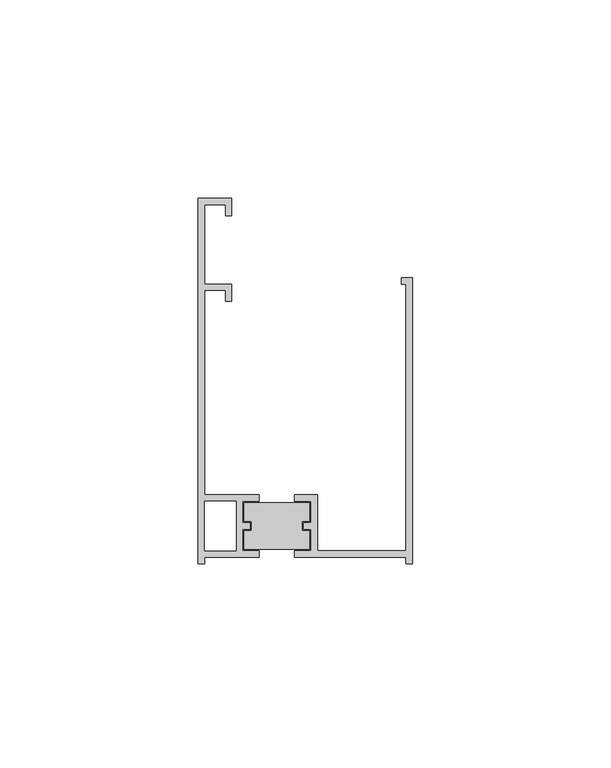
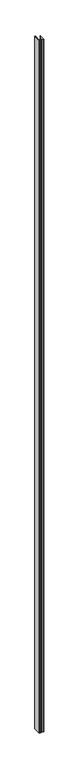
"""IFC4 building model written with IfcOpenShell, lengths in millimetres: proxy geometry, Generic Models 2:Generic Models 2:310765:Generic Models 2:310765 : Generic Models 2:Generic Models 2:310765:60 : Generic Models 2:Generic Models 2:310765:Generic Models 2:310765 : Generic Models 2:Generic Models 2:310765:300385."""

from ifc_helpers import new_model, si_unit, origin, origin_with_axes, place, context, project, spatial, polyline, outline, extrude, source, transform, mapped, element, save


def generic_models_ff3dd308(model_context):
    return source(origin(), model_context, "Body", "SweptSolid", [
        extrude(outline(polyline([(667633.5969099, -465596.2158643), (667633.5969099, -465600.9133629), (667631.6714944, -465600.9133629), (667631.6714944, -465603.2946129), (667633.5969099, -465603.2946129), (667633.5969099, -465607.9921116), (667617.0446537, -465607.9921116), (667617.0446537, -465603.2946129), (667618.9700691, -465603.2946129), (667618.9700691, -465600.9133629), (667617.0446537, -465600.9133629), (667617.0446537, -465596.2158643), (667633.5969099, -465596.2158643)])), origin_with_axes(), (0.0, 0.0, 1.0), 8775.8734497),
        extrude(outline(polyline([(667613.9760152, -465519.5639866), (667613.9760152, -465523.9513131), (667612.3885152, -465523.9513131), (667612.3885152, -465521.1514866), (667607.1171437, -465521.1514866), (667607.1171437, -465541.1514866), (667613.9760152, -465541.1514866), (667613.9760152, -465545.5388131), (667612.3885152, -465545.5388131), (667612.3885152, -465542.7389866), (667607.1171437, -465542.7389866), (667607.1171437, -465594.2314893), (667620.8149662, -465594.2314893), (667620.8149662, -465595.8189893), (667616.6477787, -465595.8189893), (667616.6477787, -465601.3102379), (667618.5731941, -465601.3102379), (667618.5731941, -465602.8977379), (667616.6477787, -465602.8977379), (667616.6477787, -465608.3889866), (667620.8149662, -465608.3889866), (667620.8149662, -465609.9764866), (667607.1171437, -465609.9764866), (667607.1171437, -465611.5639866), (667605.5296437, -465611.5639866), (667605.5296437, -465519.5639866), (667613.9760152, -465519.5639866)]), holes=[polyline([(667607.1171437, -465595.8189893), (667607.1171437, -465608.3889866), (667615.0602787, -465608.3889866), (667615.0602787, -465595.8189893), (667607.1171437, -465595.8189893)])]), origin_with_axes(), (0.0, 0.0, 1.0), 8775.8734497),
        extrude(outline(polyline([(667657.9421437, -465611.5639866), (667657.9421437, -465609.9764866), (667629.8265974, -465609.9764866), (667629.8265974, -465608.3889866), (667633.9937849, -465608.3889866), (667633.9937849, -465602.8977379), (667632.0683694, -465602.8977379), (667632.0683694, -465601.3102379), (667633.9937849, -465601.3102379), (667633.9937849, -465595.8189893), (667629.8265974, -465595.8189893), (667629.8265974, -465594.2314893), (667635.5812849, -465594.2314893), (667635.5812849, -465608.3889866), (667657.9421437, -465608.3889866), (667657.9421437, -465541.1514866), (667656.8145537, -465541.1514866), (667656.8145537, -465539.5639866), (667659.5296437, -465539.5639866), (667659.5296437, -465611.5639866), (667657.9421437, -465611.5639866)])), origin_with_axes(), (0.0, 0.0, 1.0), 8775.8734497),
    ])


if __name__ == "__main__":
    model = new_model("IFC4")
    model_context = context("Model", 3, world=origin())
    ifc_project = project(units=[si_unit("LENGTHUNIT", "METRE", prefix="MILLI")], contexts=[model_context])
    site = spatial("IfcSite", under=ifc_project)
    building = spatial("IfcBuilding", under=site)
    placement = place(None, origin())
    generic_models_shape = generic_models_ff3dd308(model_context)
    element("IfcBuildingElementProxy", 1, Name="Generic Models 2:Generic Models 2:310765:Generic Models 2:310765 : Generic Models 2:Generic Models 2:310765:60 : Generic Models 2:Generic Models 2:310765:Generic Models 2:310765 : Generic Models 2:Generic Models 2:310765:300385", ObjectType="Generic Models 2:Generic Models 2:310765:Generic Models 2:310765 : Generic Models 2:Generic Models 2:310765:60 : Generic Models 2:Generic Models 2:310765:Generic Models 2:310765 : Generic Models 2:Generic Models 2:310765:300385", at=placement, inside=building, context=model_context, shape_type="MappedRepresentation", body=[
        mapped(generic_models_shape, transform((0.0, 0.0, 0.0), x_axis=(1.0, 0.0, 0.0), y_axis=(0.0, 1.0, 0.0), z_axis=(0.0, 0.0, 1.0))),
    ])
    save(model, "model.ifc")

# Revit data of these elements
# Type "Generic Models 2:Generic Models 2:310765:Generic Models 2:310765 : Generic Models 2:Generic Models 2:310765:60 : Generic Models 2:Generic Models 2:310765:Generic Models 2:310765 : Generic Models 2:Generic Models 2:310765:300385"
#   NameOverride = "Generic Models 2:Generic Models 2:310765:Generic Models 2:310765 : Generic Models 2:Generic Models 2:310765:300385"
#   ObjectTypeOverride = "Generic Models 2:310765 : Generic Models 2:Generic Models 2:310765"
#   Reference = "Generic Models 2"
#   Tag = "300385"
# Element 1 (IfcBuildingElementProxy, "Generic Models 2:Generic Models 2:310765:Generic Models 2:310765 : Generic Models 2:Generic Models 2:310765:60 : Generic Models 2:Generic Models 2:310765:Generic Models 2:310765 : Generic Models 2:Generic Models 2:310765:300385")
#   Materials on its faces: "THERMAL BROKEN ALUMINUM STOREFRONT FOR POLYCARBONATE"
# Materials
#   "THERMAL BROKEN ALUMINUM STOREFRONT FOR POLYCARBONATE": class "Unassigned", colour RGB 244 244 244, transparency 0, Keynote = "M07611300.01", Cost = 0
